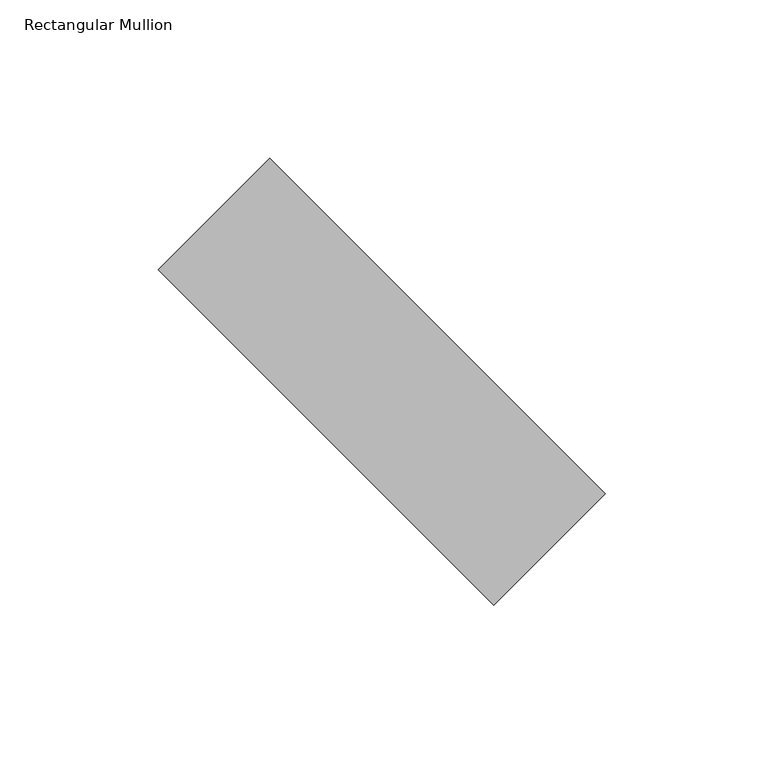
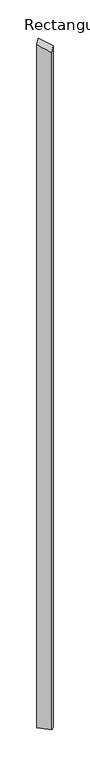
"""IFC4 building model written with IfcOpenShell, lengths in millimetres: member geometry, Rectangular Mullion : tilted mullions."""

from ifc_helpers import new_model, si_unit, origin, place, context, project, spatial, faceted_brep, source, transform, mapped, element, save


def rectangular_mullion_989ad972(model_context):
    return source(origin(), model_context, "Body", "Brep", [
        faceted_brep([(-35.3553391, 70.7106781, -7999.5991341), (70.7106781, -35.3553391, -7999.5991341), (35.3553391, -70.7106781, -7999.5991341), (-70.7106781, 35.3553391, -7999.5991341), (-70.7106781, 35.3553391, 9.9898148), (-35.3553391, 70.7106781, 55.0457921), (35.3553391, -70.7106781, -55.0457921), (70.7106781, -35.3553391, -9.9898148)], [[[0, 1, 2, 3]], [[4, 5, 0, 3]], [[6, 4, 3, 2]], [[7, 6, 2, 1]], [[5, 7, 1, 0]], [[5, 4, 6, 7]]]),
    ])


if __name__ == "__main__":
    model = new_model("IFC4")
    model_context = context("Model", 3, world=origin())
    ifc_project = project(units=[si_unit("LENGTHUNIT", "METRE", prefix="MILLI")], contexts=[model_context])
    site = spatial("IfcSite", under=ifc_project)
    building = spatial("IfcBuilding", under=site)
    placement = place(None, origin())
    rectangular_mullion_shape = rectangular_mullion_989ad972(model_context)
    element("IfcMember", 1, ObjectType="Rectangular Mullion : tilted mullions", at=placement, inside=building, context=model_context, shape_type="MappedRepresentation", body=[
        mapped(rectangular_mullion_shape, transform((0.0, 0.0, 0.0), x_axis=(1.0, 0.0, 0.0), y_axis=(0.0, 1.0, 0.0), z_axis=(0.0, 0.0, 1.0))),
    ])
    save(model, "model.ifc")

# Revit data of these elements
# Type "Rectangular Mullion : tilted mullions"
#   built-in parameter 1007304 = 0.492126 (stored number, unit not read)
#   built-in parameter 1007301 = 0.082021 (stored number, unit not read)
#   built-in parameter 1007300 = 0.082021 (stored number, unit not read)
# Element 1 (IfcMember, "Rectangular Mullion : tilted mullions")
#   Materials on its faces: "Aluminum"
# Materials
#   "Aluminum": class "Metal", colour RGB 244 244 244, transparency 0, Description = "Aluminum 6061", Cost = 0
